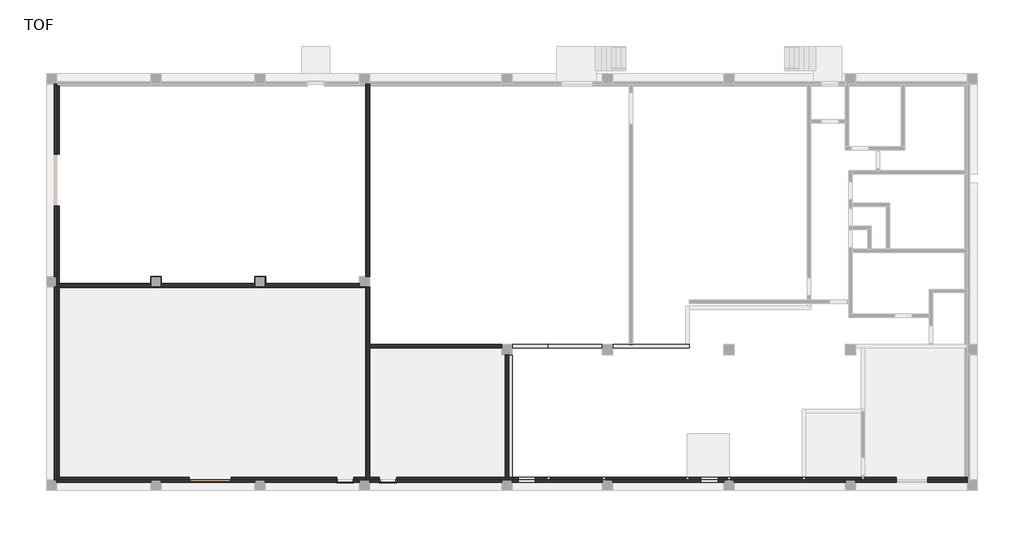
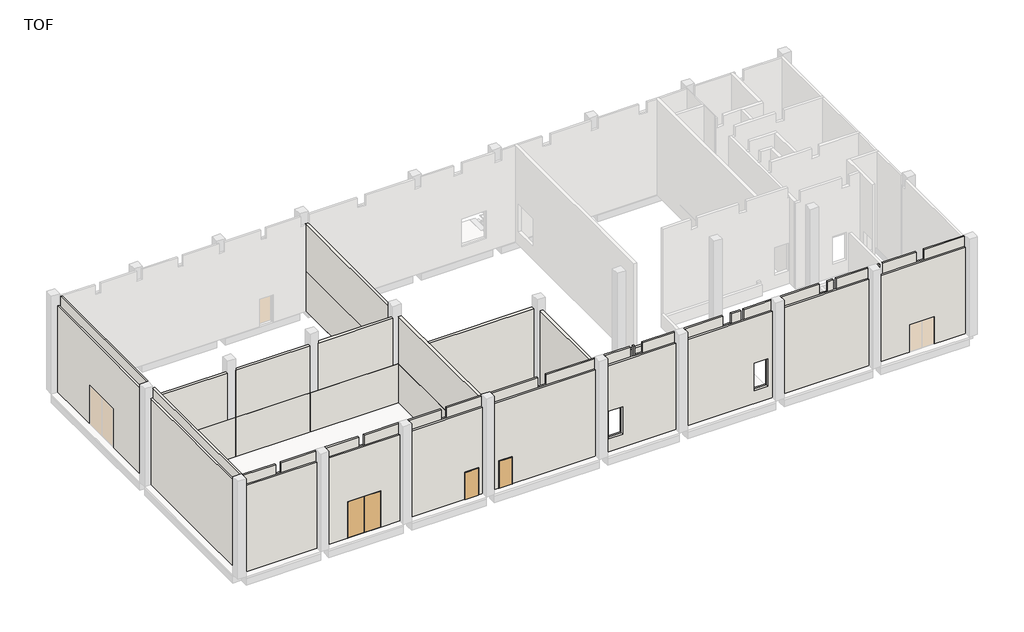
# One storey, part 1 of 4: 21 walls, 3 doors.
# Revit data of these elements (continued)
# Project information
#   H_Seismic Condition = "A as per ASCE 7-10"
#   H_Soil Condition = "C as per ASCE 7-10"
#   H_Basic Wind Speed = "58.3m/s ASCE7-10"
#   Building Name = "설퍼로딩컨트롤빌딩"
#   H_DS Project Code = "FAASA2302"
#   H_Project Abbreviation = "SACE2"
#   H_Project Division = "화공"
#   H_Project Finish = "2027-03-05"
#   H_Project Location = "Jafurah, Saudi Arabia"
#   H_Project Start = "2024-01-03"
#   H_Project Type = "EPC"
#   H_Smart Code = "FAASA2302"
#   Project Issue Date = "Issue Date"
#   Project Status = "Project Status"
#   Client Name = "Owner"
#   Project Address = "Enter address here"
#   Project Name = "자푸라2"
#   Project Number = "0001"
# Grids (mm)
#   "18": line (36400, 29277.337) -> (36400, -4496.638)
#   "C": line (-3860.098, 12199.521) -> (22160.842, 12199.521)
#   "1": line (0, 29277.337) -> (0, -4496.638)
#   "2": line (6000, 29277.337) -> (6000, -4496.638)
#   "D": line (-3860.098, 23899.521) -> (59043.988, 23899.521)
#   "B": line (-3860.098, 8299.521) -> (59043.988, 8299.521)
#   "A": line (-3860.098, 499.521) -> (59043.988, 499.521)
#   "3": line (12000, 29277.337) -> (12000, -4496.638)
#   "4": line (18000, 29277.337) -> (18000, -4496.638)
#   "5": line (26200, 29277.337) -> (26200, -4496.638)
#   "6": line (32000, 29277.337) -> (32000, -4496.638)
#   "7": line (39000, 29277.337) -> (39000, -4496.638)
#   "8": line (46000, 29277.337) -> (46000, -4496.638)
#   "9": line (53000, 29277.337) -> (53000, -4496.638)
#   "X11": line (55259.645, 21449.521) -> (42900, 21449.521)
#   "X12": line (55259.645, 19899.521) -> (45500, 19899.521)
#   "X13": line (55259.645, 18499.521) -> (45500, 18499.521)
#   "X14": line (55259.645, 16649.521) -> (45500, 16649.521)
#   "X15": line (55259.645, 13999.521) -> (45500, 13999.521)
#   "X18": line (46700, -1149.47) -> (46700, 6768.825)
#   "X19": line (55259.645, 6699.521) -> (42900, 6699.521)
#   "X21": line (55259.645, 4749.521) -> (38600, 4749.521)
#   "X23": line (43300, -1149.47) -> (43300, 8899.521)
#   "X24": line (36600, -1149.47) -> (36600, 11674.521)
#   "X25": line (28600, -1149.47) -> (28600, 8899.521)
#   "X26": line (42900, 18149.521) -> (59043.988, 18149.521)
#   "X27": line (55259.645, 10849.521) -> (36075, 10849.521)
#   "X28": line (-3860.098, 25749.521) -> (59043.988, 25749.521)
#   "X16": line (55259.645, 11049.521) -> (36075, 11049.521)
#   "10": line (3000, 29277.337) -> (3000, -4496.638)
#   "11": line (9000, 29277.337) -> (9000, -4496.638)
#   "12": line (15000, 29277.337) -> (15000, -4496.638)
#   "13": line (22100, 29277.337) -> (22100, -4496.638)
#   "14": line (29100, 29277.337) -> (29100, -4496.638)
#   "15": line (35500, 29277.337) -> (35500, -4496.638)
#   "16": line (42500, 29277.337) -> (42500, -4496.638)
#   "17": line (49500, 29277.337) -> (49500, -4496.638)
#   "X29": line (-3860.098, -1337.479) -> (59043.988, -1337.479)
#   "X17": line (55259.645, 10249.521) -> (45500, 10249.521)
# Type "Double Door_Steel : H_DR_AR_B12_Double Door_Steel_W2400xH2800"
#   Type Mark = "429"
#   프레임 = ""
#   철물 = ""
#   유리/마감 = ""
#   위치/개소 = ""
#   부호 = "1/SD"
#   문번호 = ""
#   문기호 = "SD"
#   Analytic Construction = "<None>"
#   Height = 2800 mm
#   Width = 2400 mm
#   Define Thermal Properties by = 1
#   문 틀 = none
#   문 = none
#   Function = (empty or 0)
#   Assembly Code = ""
#   Wall Closure = (empty or 0)
# Type "Single Door_Steel : H_DR_AR_B12_Single Door_Steel_W1000xH2100"
#   Type Mark = "SD"
#   Analytic Construction = "<None>"
#   프레임 투영 외부. = 25 mm
#   프레임 투영 내부. = 25 mm
#   프레임 폭 = 75 mm
#   Height = 2100 mm
#   Width = 1000 mm
#   Define Thermal Properties by = 1
#   문 패널 = none
#   문 프레임 = none
#   Function = (empty or 0)
#   Wall Closure = (empty or 0)
# Type "H_WA_AR_B02_Ext Wall_RC T150"
#   Type Comments = ""
#   Layers, outside or top first: 150 mm "Concrete - Cast-in-Place Concrete - 35 MPa" (function 1)
# Type "H_WA_AR_B02_Int Wall_Block T200"
#   Type Comments = ""
#   Layers, outside or top first: 200 mm "00_Masonry_Conc. Block" (function 1)
# Type "H_WA_AR_B07_Int Wall_Plaster T12"
#   Type Comments = ""
#   Layers, outside or top first: 12 mm "Plaster" (function 2)
# Type "H_WA_AR_B02_Ext Wall_1L Gypsum_Mineral Wool_T110"
#   Type Comments = "구조_콘크리트"
#   Layers, outside or top first: 110 mm "Rock Wool" (function 2); 16 mm "Gypsum Wall Board" (function 1)
# Type "H_WA_AR_B02_Int Wall_RC"
#   Type Comments = ""
#   Layers, outside or top first: 200 mm "Concrete - Cast-in-Place Concrete - 35 MPa" (function 1)
# Element 1 (IfcDoor, "Double Door_Steel : H_DR_AR_B12_Double Door_Steel_W2400xH2800")
#   H_Door Style Name = "Steel Door_Double_Transsom"
#   H_Door_Frame = "Steel"
#   H_Door_Leaf = "Steel"
#   H_Door_Vision = "N.A"
#   H_Door_Panic = "N.A"
#   H_Door_Style Remark = ""
#   H_Door_Fire Rating = "NA/0.5/1.0\n/1.5/2.0"
#   H_Door Style No = DDT11
#   Phase Created = New Construction
# Elements 2, 3 (IfcDoor, "Single Door_Steel : H_DR_AR_B12_Single Door_Steel_W1000xH2100")
#   H_Door Style Name = "Steel Door_Single"
#   H_Door_Frame = "Steel"
#   H_Door_Leaf = "Steel"
#   H_Door_Vision = "N.A"
#   H_Door_Panic = "N.A"
#   H_Door_Style Remark = "Steel Door w/ Steel Frame"
#   H_Door_Fire Rating = "NA/0.5/1.0\n/1.5/2.0"
#   H_Door Style No = SD11
#   Phase Created = New Construction
# Elements 4, 5 (IfcWall, "H_WA_AR_B02_Ext Wall_RC T150")
#   H_Wall Style Name = "Gypsum Board Wall+Mineral Wool Insulation w/ Air Space+Concrete Wall+Acrylic Emulsion Paint on Fair Faced Concrete"
#   H_Wall-Base Material-1 = "1-Layer Gypsum Board"
#   H_Wall-Base Material-2 = "Mineral Wool (Rock Wool)+Air Space"
#   H_Wall_Finish-In = "Acrylic Emulsion Paint"
#   H_Wall_Base Material-3 = "Concrete Wall"
#   H_Wall_Finish-Ex = "Acrylic Emulsion Paint on Fair Faced Concrete"
#   H_Wall_Style Remark = "WM : Plasterboard Dry Liner System (A04AS176-00001~00009)\n        - Gypsum Board + Insulation\n        (Gypsumboard THK=9.5 & 12.5 & 16 mm)"
#   Top Offset = 0 mm
#   Base Offset = 0 mm
#   wall height = 7500 mm
#   H_Wall Style No = EW11
#   Phase Created = New Construction
#   Base Constraint = TOF
#   Top Constraint = TOC
#   Materials on its faces: "Concrete - Cast-in-Place Concrete - 35 MPa"
# Elements 6, 7, 8 (IfcWall, "H_WA_AR_B02_Int Wall_Block T200")
#   H_Wall Style Name = "Block Wall"
#   H_Wall-Base Material-1 = "Concrete Block"
#   H_Wall-Base Material-2 = ""
#   H_Wall_Finish-In = "Acrylic Emulsion Paint on Cement Plaster"
#   H_Wall_Base Material-3 = ""
#   H_Wall_Finish-Ex = "Acrylic Emulsion Paint on Cement Plaster"
#   H_Wall_Style Remark = "WM : Reinforced Concrete Block\n     50mm<THK≤100mm / 100mm<THK≤200mm / 200mm<THK"
#   Top Offset = 0 mm
#   Base Offset = 0 mm
#   wall height = 7500 mm
#   H_Wall Style No = IW21
#   Phase Created = New Construction
#   Base Constraint = TOF
#   Top Constraint = TOC
#   Materials on its faces: "00_Masonry_Conc. Block"
# Elements 9, 10, 11, 12, 13, 14, 15, 16, 17, 20, 21 (IfcWall, "H_WA_AR_B07_Int Wall_Plaster T12")
#   Top Offset = 0 mm
#   Base Offset = 0 mm
#   Unconnected Height = 3000 mm
#   wall height = 3000 mm
#   Phase Created = New Construction
#   Base Constraint = TOF
#   Materials on its faces: "Plaster"
# Elements 18, 19 (IfcWall, "H_WA_AR_B02_Ext Wall_1L Gypsum_Mineral Wool_T110")
#   Top Offset = 0 mm
#   Base Offset = 0 mm
#   wall height = 7500 mm
#   Phase Created = New Construction
#   Base Constraint = TOF
#   Top Constraint = TOC
#   Materials on its faces: "Rock Wool", "Gypsum Wall Board"
# Elements 22, 23 (IfcWall, "H_WA_AR_B02_Int Wall_RC")
#   Top Offset = 0 mm
#   Base Offset = 0 mm
#   wall height = 1000 mm
#   Phase Created = New Construction
#   Base Constraint = TOF
#   Top Constraint = TOF2
#   Materials on its faces: "Concrete - Cast-in-Place Concrete - 35 MPa"
# Element 24 (IfcWall, "H_WA_AR_B02_Int Wall_Block T200")
#   H_Wall Style Name = "Block Wall"
#   H_Wall-Base Material-1 = "Concrete Block"
#   H_Wall-Base Material-2 = ""
#   H_Wall_Finish-In = "Acrylic Emulsion Paint on Cement Plaster"
#   H_Wall_Base Material-3 = ""
#   H_Wall_Finish-Ex = "Acrylic Emulsion Paint on Cement Plaster"
#   H_Wall_Style Remark = "WM : Reinforced Concrete Block\n     50mm<THK≤100mm / 100mm<THK≤200mm / 200mm<THK"
#   Top Offset = 0 mm
#   Base Offset = 0 mm
#   wall height = 7500 mm
#   Phase Created = New Construction
#   Base Constraint = TOF
#   Top Constraint = TOC
#   Materials on its faces: "00_Masonry_Conc. Block"
# Materials
#   "Concrete - Cast-in-Place Concrete - 35 MPa": class "Concrete", colour RGB 192 192 192, transparency 0, Cost = 0
#   "00_Masonry_Conc. Block": class "Concrete", colour RGB 180 180 180, transparency 0, Description = "Conc. Block", Cost = 0, Image = Brick_Uniform_12inch_Running_Gray.png
#   "Plaster": class "Generic", colour RGB 249 249 249, transparency 0, Description = "Plaster", Cost = 0
#   "Rock Wool": class "Generic", colour RGB 120 120 120, transparency 0, Description = "Rock Wool", Cost = 0
#   "Gypsum Wall Board": class "Generic", colour RGB 171 170 168, transparency 0, Description = "Gypsum Wall Board", Cost = 0
